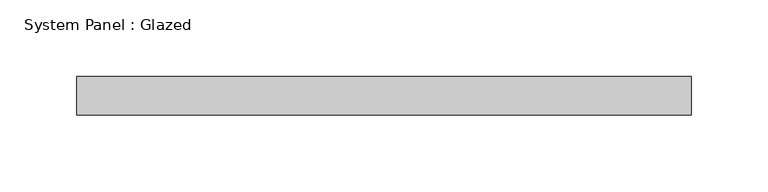
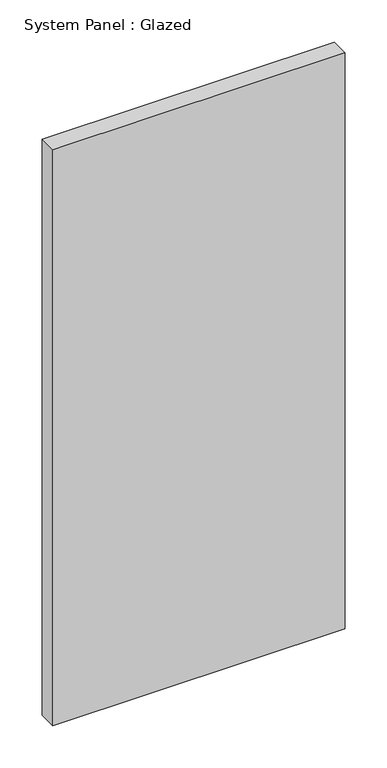
"""IFC4 building model written with IfcOpenShell, lengths in millimetres: plate geometry, System Panel : Glazed."""

from ifc_helpers import new_model, si_unit, origin, origin_with_axes, place, context, project, spatial, polyline, outline, extrude, source, transform, mapped, element, save


def system_panel_glazed_16830f23(model_context):
    return source(origin(), model_context, "Body", "SweptSolid", [
        extrude(outline(polyline([(200.0, 24.5), (-200.0, 24.5), (-200.0, 49.5), (200.0, 49.5), (200.0, 24.5)])), origin_with_axes(), (0.0, 0.0, 1.0), 833.3333333),
    ])


if __name__ == "__main__":
    model = new_model("IFC4")
    model_context = context("Model", 3, world=origin())
    ifc_project = project(units=[si_unit("LENGTHUNIT", "METRE", prefix="MILLI")], contexts=[model_context])
    site = spatial("IfcSite", under=ifc_project)
    building = spatial("IfcBuilding", under=site)
    placement = place(None, origin())
    system_panel_glazed_shape = system_panel_glazed_16830f23(model_context)
    element("IfcPlate", 1, ObjectType="System Panel : Glazed", at=placement, inside=building, context=model_context, shape_type="MappedRepresentation", body=[
        mapped(system_panel_glazed_shape, transform((0.0, 0.0, 0.0), x_axis=(1.0, 0.0, 0.0), y_axis=(0.0, 1.0, 0.0), z_axis=(0.0, 0.0, 1.0))),
    ])
    save(model, "model.ifc")

# Revit data of these elements
# Element 1 (IfcPlate, "System Panel : Glazed")
#   Materials on its faces: "Glass"
# Materials
#   "Glass": class "Glass", colour RGB 218 227 224, transparency 0.85, Description = "Soda Lime Glass", Cost = 0
